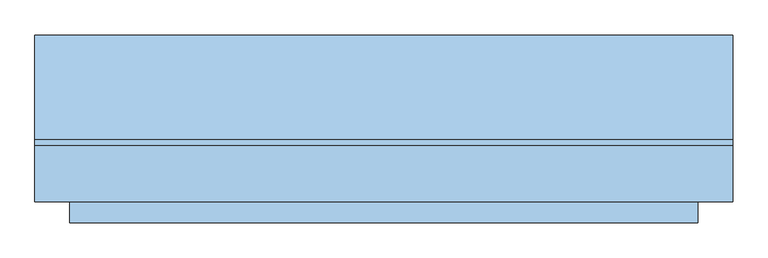
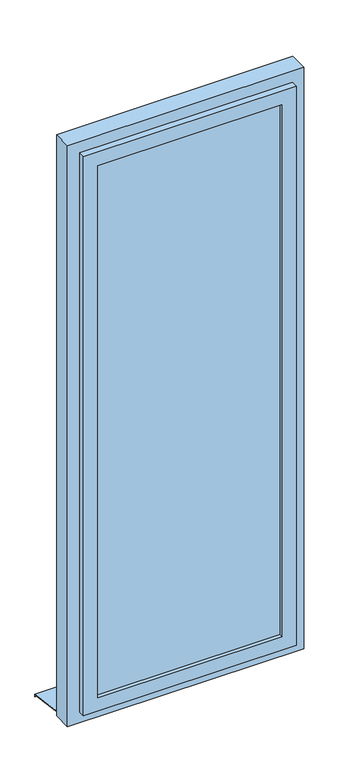
"""IFC4 building model written with IfcOpenShell, lengths in millimetres: window geometry, Fenstertür 1-flg : 1.80 x  1."""

from ifc_helpers import new_model, si_unit, frame, origin, place, context, project, spatial, polyline, outline, extrude, faceted_brep, source, transform, mapped, element, save


def window_4f3e8dcf(model_context):
    return source(origin(), model_context, "Body", "SolidModel", [
        extrude(outline(polyline([(2600.0, 500.0), (2600.0, -500.0), (0.0, -500.0), (0.0, 500.0), (2600.0, 500.0)]), holes=[polyline([(2520.0, 420.0), (80.0, 420.0), (80.0, -420.0), (2520.0, -420.0), (2520.0, 420.0)])]), frame((0.0, -58.6893832, 0.0), z_axis=(0.0, 1.0, 0.0), x_axis=(0.0, 0.0, 1.0)), (0.0, 0.0, 1.0), 80.0),
        faceted_brep([(450.0, -58.6893832, 2550.0), (450.0, -88.6893832, 2550.0), (450.0, -88.6893832, 50.0), (450.0, -58.6893832, 50.0), (-450.0, -88.6893832, 2550.0), (-450.0, -88.6893832, 50.0), (390.0, -88.6893832, 110.0), (-390.0, -88.6893832, 110.0), (-390.0, -88.6893832, 2490.0), (390.0, -88.6893832, 2490.0), (-450.0, -58.6893832, 50.0), (-450.0, -58.6893832, 2550.0), (420.0, -58.6893832, 2520.0), (-420.0, -58.6893832, 2520.0), (-420.0, -58.6893832, 80.0), (420.0, -58.6893832, 80.0), (420.0, -28.6893832, 2520.0), (420.0, -28.6893832, 80.0), (-420.0, -28.6893832, 80.0), (-420.0, -28.6893832, 2520.0), (390.0, -28.6893832, 2490.0), (-390.0, -28.6893832, 2490.0), (-390.0, -28.6893832, 110.0), (390.0, -28.6893832, 110.0)], [[[0, 1, 2, 3]], [[1, 4, 5, 2], [6, 7, 8, 9]], [[3, 2, 5, 10]], [[3, 10, 11, 0], [12, 13, 14, 15]], [[16, 12, 15, 17]], [[17, 15, 14, 18]], [[17, 18, 19, 16], [20, 21, 22, 23]], [[9, 20, 23, 6]], [[6, 23, 22, 7]], [[10, 5, 4, 11]], [[18, 14, 13, 19]], [[7, 22, 21, 8]], [[11, 4, 1, 0]], [[19, 13, 12, 16]], [[8, 21, 20, 9]]]),
        extrude(outline(polyline([(31.3327711, 20.0), (180.0, 0.0), (180.0, -10.0), (178.0, -10.0), (178.0, -1.6395366), (31.1346891, 18.0), (21.3106168, 18.0), (21.3106168, 20.0), (31.3327711, 20.0)])), frame((-500.0, 0.0, 0.0), z_axis=(1.0, 0.0, 0.0), x_axis=(0.0, 1.0, 0.0)), (0.0, 0.0, 1.0), 1000.0),
        extrude(outline(polyline([(390.0, -73.6893832), (-390.0, -73.6893832), (-390.0, -43.6893832), (390.0, -43.6893832), (390.0, -73.6893832)])), frame((0.0, 0.0, 110.0), z_axis=(0.0, 0.0, 1.0), x_axis=(1.0, 0.0, 0.0)), (0.0, 0.0, 1.0), 2380.0),
    ])


if __name__ == "__main__":
    model = new_model("IFC4")
    model_context = context("Model", 3, world=origin())
    ifc_project = project(units=[si_unit("LENGTHUNIT", "METRE", prefix="MILLI")], contexts=[model_context])
    site = spatial("IfcSite", under=ifc_project)
    building = spatial("IfcBuilding", under=site)
    placement = place(None, origin())
    window_shape = window_4f3e8dcf(model_context)
    element("IfcWindow", 1, ObjectType="Fenstertür 1-flg : 1.80 x  1", at=placement, inside=building, context=model_context, shape_type="MappedRepresentation", body=[
        mapped(window_shape, transform((0.0, 0.0, 0.0), x_axis=(1.0, 0.0, 0.0), y_axis=(0.0, 1.0, 0.0), z_axis=(0.0, 0.0, 1.0))),
    ])
    save(model, "model.ifc")

# Revit data of these elements
# Type "Fenstertür 1-flg : 1.80 x  1"
#   Type Mark = "73"
#   Operation = "SinglePanel"
#   Construction Type Id = "GSP4R"
#   Keynote = "16.05.01"
#   Analytic Construction = "1/8 Zoll Pilkington-Verglasung einfach"
#   Visual Light Transmittance = 0.9
#   Thermal Resistance (R) = 0.1491 (m²·K)/W
#   Solar Heat Gain Coefficient = 0.86
#   Rough Width = 1.000 m
#   Rough Height = 2.600 m
#   Heat Transfer Coefficient (U) = 6.7069 W/(m²·K)
#   Rahmentiefe = 0.080 m
#   Rahmenhöhe - unten = 0.080 m
#   Rahmenhöhe - oben = 0.080 m
#   Rahmenbreite = 0.080 m
#   Height = 2.600 m
#   Tiefe Flügel = 0.060 m
#   Flügelbreite = 0.060 m
#   Einbautiefe (von außen) [instance default] = 0.080 m
#   Width = 1.000 m
#   Kippflügel [instance default] = yes
#   Drehflügel im Grundriss darstellen [instance default] = yes
#   Drehflügel 1 [instance default] = yes
#   Rahmen 1 [instance default] = none
#   Glas [instance default] = none
#   Flügel [instance default] = none
#   Fensterbank Außenseite [instance default] = none
#   Wall Closure = (empty or 0)
# Element 1 (IfcWindow, "Fenstertür 1-flg : 1.80 x  1")
#   Einbautiefe (von außen) = 0.128689 m
#   Materials on its faces: "Kunststoff - Weiß", "Glas"
# Materials
#   "Kunststoff - Weiß": class "Kunststoff", colour RGB 249 249 249, transparency 0, Cost = 0
#   "Glas": class "Glas", colour RGB 0 0 255, transparency 0.75, Comments = "Render-Darstellung nicht aktualisiert ", Cost = 0
